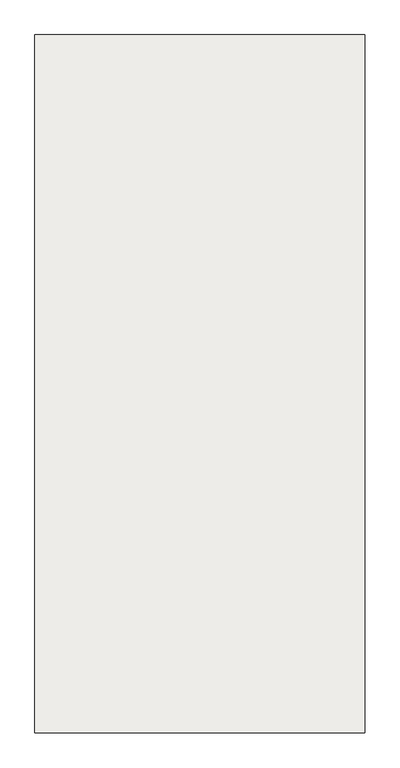
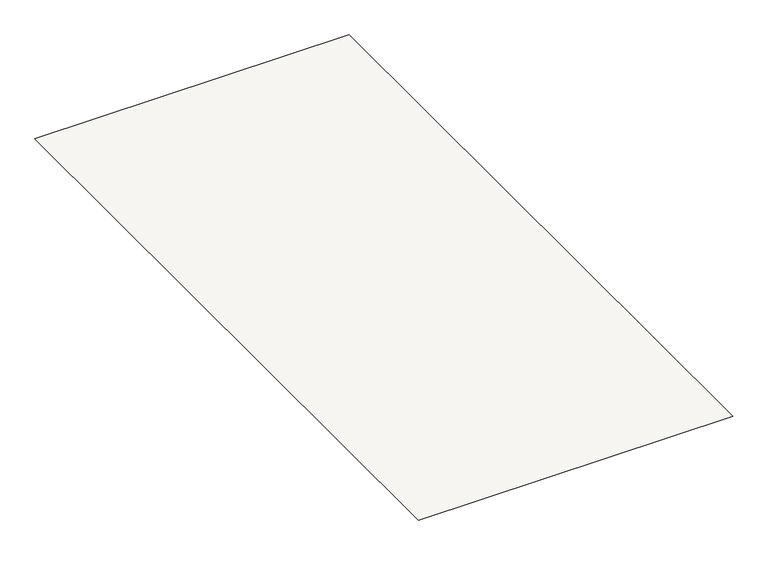
"""IFC4 building model written with IfcOpenShell, lengths in millimetres: slab geometry, EQUIMENT FDN.2 : FTS211_EF_EF2."""

from ifc_helpers import new_model, si_unit, origin, place, context, project, spatial, faceted_brep, source, transform, mapped, element, save


def slab_9e7bc1f9(model_context):
    return source(origin(), model_context, "Body", "Brep", [
        faceted_brep([(44894.0, 29249.5208589, 199.9720055), (44894.0, 25149.5208589, 199.9720055), (43294.0, 25149.5208589, 199.9720055), (43294.0, 29249.5208589, 199.9720055), (42974.0, 29569.5208589, 399.9720055), (45214.0, 29569.5208589, 399.9720055), (42974.0, 24829.5208589, 399.9720055), (45214.0, 24829.5208589, 399.9720055)], [[[0, 1, 2, 3]], [[0, 3, 4, 5]], [[3, 2, 6, 4]], [[2, 1, 7, 6]], [[1, 0, 5, 7]], [[5, 4, 6, 7]]]),
    ])


if __name__ == "__main__":
    model = new_model("IFC4")
    model_context = context("Model", 3, world=origin())
    ifc_project = project(units=[si_unit("LENGTHUNIT", "METRE", prefix="MILLI")], contexts=[model_context])
    site = spatial("IfcSite", under=ifc_project)
    building = spatial("IfcBuilding", under=site)
    placement = place(None, origin())
    slab_shape = slab_9e7bc1f9(model_context)
    element("IfcSlab", 1, ObjectType="EQUIMENT FDN.2 : FTS211_EF_EF2", at=placement, inside=building, context=model_context, shape_type="MappedRepresentation", body=[
        mapped(slab_shape, transform((0.0, 0.0, 0.0), x_axis=(1.0, 0.0, 0.0), y_axis=(0.0, 1.0, 0.0), z_axis=(0.0, 0.0, 1.0))),
    ])
    save(model, "model.ifc")

# Revit data of these elements
# Element 1 (IfcSlab, "EQUIMENT FDN.2 : FTS211_EF_EF2")
#   Materials on its faces: "A03AD032-00010_Structural Concrete_UG_20-24MPa"
# Materials
#   "A03AD032-00010_Structural Concrete_UG_20-24MPa": class "Concrete", colour RGB 176 176 176, transparency 0, Keynote = "09910.A1", Description = "Substructure Concrete / Cement Type-1 / 24MPa", Cost = 0
